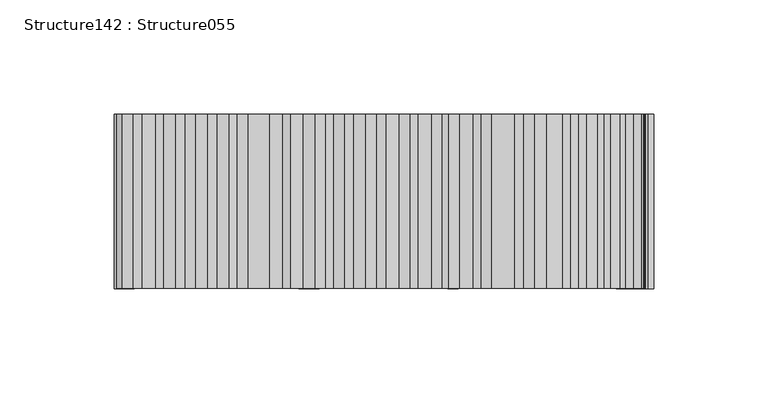
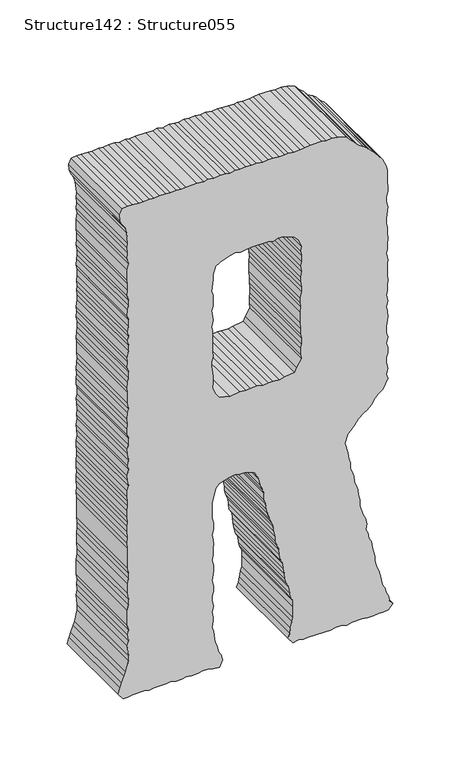
"""IFC4 building model written with IfcOpenShell, lengths in millimetres: proxy geometry, Structure142 : Structure055."""

from ifc_helpers import new_model, si_unit, frame, origin, place, context, project, spatial, polyline, outline, extrude, source, transform, mapped, element, save


def structure142_structure055_61f402d9(model_context):
    return source(origin(), model_context, "Body", "SweptSolid", [
        extrude(outline(polyline([(3899.7046941, -44803.696828), (3903.2059411, -44804.280904), (3907.888177, -44804.280904), (3918.4480792, -44803.1063335), (3923.1319197, -44804.280904), (3927.8077372, -44804.280904), (3932.4899731, -44803.1063335), (3936.0345445, -44803.1063335), (3941.8753048, -44803.696828), (3951.2606365, -44803.696828), (3955.360401, -44804.280904), (3962.9774586, -44807.7965925), (3967.6789497, -44811.3138855), (3970.5768654, -44813.6469805), (3974.1214368, -44817.7563726), (3977.6194746, -44820.679962), (3979.9621971, -44823.6244112), (3982.8793681, -44828.2986241), (3987.0048063, -44831.8143126), (3989.9460463, -44835.3396286), (3994.0233463, -44838.8601309), (3996.390138, -44845.8834848), (3997.5486624, -44851.1497967), (3996.9645864, -44855.8432649), (3997.5486624, -44859.9414248), (3997.5486624, -44869.9012049), (3996.9645864, -44874.594673), (3996.390138, -44878.1023385), (3996.390138, -44883.9703771), (3996.9645864, -44888.64459), (3996.390138, -44891.5890392), (3996.390138, -44896.2616475), (3996.9645864, -44902.1296862), (3996.9645864, -44905.6469792), (3996.390138, -44910.3404474), (3997.5486624, -44916.1908354), (3996.9645864, -44920.3002275), (3997.5486624, -44924.9824634), (3996.9645864, -44930.2487754), (3997.5486624, -44934.3485398), (3996.390138, -44939.042008), (3996.9645864, -44942.559301), (3997.5486624, -44947.2511646), (3996.390138, -44952.5190811), (3997.5486624, -44957.7934161), (3996.390138, -44961.3107092), (3996.9645864, -44967.1610972), (3996.9645864, -44976.5448243), (3996.390138, -44981.2286648), (3996.9645864, -44984.7443532), (3996.390138, -44990.0138744), (3996.9645864, -44994.1232665), (3996.9645864, -44999.3976015), (3996.390138, -45004.0798374), (3996.9645864, -45008.1715789), (3996.390138, -45013.4555415), (3996.390138, -45016.9664161), (3996.9645864, -45022.8312455), (3996.9645864, -45026.922987), (3996.390138, -45031.6164552), (3991.6806238, -45033.9655961), (3986.4046842, -45033.3847293), (3981.7208437, -45031.6164552), (3978.2035506, -45029.2753372), (3973.5197101, -45028.1007667), (3963.5615346, -45026.922987), (3959.4617701, -45027.5166907), (3954.7506513, -45026.922987), (3949.4923624, -45027.5166907), (3944.8165449, -45026.3485386), (3939.5325823, -45027.5166907), (3930.1745289, -45027.5166907), (3926.6492128, -45026.922987), (3920.7908018, -45026.922987), (3916.0909152, -45027.5166907), (3911.4054701, -45026.3485386), (3906.7328618, -45026.3485386), (3903.2059411, -45026.922987), (3897.3475301, -45027.5166907), (3893.822214, -45026.3485386), (3887.9621984, -45026.3485386), (3883.2863809, -45026.922987), (3878.5784713, -45026.3485386), (3875.0772243, -45026.922987), (3870.4030114, -45026.3485386), (3865.7015202, -45026.3485386), (3859.8591552, -45027.5166907), (3855.7353217, -45026.922987), (3850.4754282, -45027.5166907), (3846.3772683, -45026.3485386), (3841.0900965, -45026.3485386), (3836.9919366, -45026.922987), (3831.732043, -45027.5166907), (3828.2163546, -45026.922987), (3818.2309008, -45026.922987), (3812.9726119, -45026.3485386), (3809.4729695, -45026.922987), (3803.5872802, -45027.5166907), (3798.9050443, -45026.922987), (3794.8309535, -45027.5166907), (3789.5293402, -45027.5166907), (3786.0280932, -45026.3485386), (3780.1616592, -45026.3485386), (3776.6427615, -45027.5166907), (3771.9605256, -45026.922987), (3766.1021146, -45026.3485386), (3761.418274, -45026.922987), (3757.8753073, -45026.3485386), (3752.6170184, -45027.5166907), (3747.9428055, -45026.922987), (3742.6748889, -45026.3485386), (3738.5574738, -45027.5166907), (3733.2991849, -45027.5166907), (3729.1737467, -45026.922987), (3725.0996559, -45026.922987), (3720.4158154, -45027.5166907), (3714.5301261, -45027.5166907), (3709.8559132, -45026.922987), (3706.3289925, -45027.5166907), (3701.6547796, -45027.5166907), (3695.786741, -45026.922987), (3691.0868544, -45027.5166907), (3686.4030139, -45026.922987), (3668.2437048, -45026.922987), (3663.5598643, -45026.3485386), (3658.8840468, -45026.3485386), (3654.1841602, -45026.922987), (3645.4262289, -45026.922987), (3639.5405396, -45026.3485386), (3634.856699, -45026.3485386), (3630.1824862, -45027.5166907), (3616.69739, -45027.5166907), (3612.0135494, -45026.3485386), (3607.8961343, -45026.922987), (3602.0280957, -45026.3485386), (3597.9540049, -45027.5166907), (3588.5702778, -45026.3485386), (3583.8864372, -45026.3485386), (3574.5107332, -45028.6912612), (3570.9854171, -45029.8674363), (3565.7094775, -45032.1989266), (3561.6257591, -45033.3847293), (3556.3417965, -45035.1337482), (3551.0658569, -45031.0243561), (3551.0658569, -45026.922987), (3551.6675836, -45022.8312455), (3551.6675836, -45012.865047), (3551.0658569, -45008.7652825), (3551.6675836, -45004.0798374), (3551.6675836, -44994.1232665), (3552.242032, -44989.4297984), (3551.0658569, -44985.3380569), (3551.0658569, -44980.6461934), (3551.6675836, -44976.5448243), (3551.0658569, -44971.8513561), (3551.6675836, -44966.5866488), (3552.242032, -44962.4852797), (3552.242032, -44958.3758876), (3551.0658569, -44953.6936516), (3550.4833855, -44947.833636), (3556.3417965, -44945.4828904), (3561.6257591, -44946.6590655), (3565.1254015, -44949.0001835), (3570.9854171, -44950.1763586), (3574.5107332, -44951.9253775), (3585.0706354, -44953.099948), (3589.1527492, -44954.2777277), (3594.4286888, -44953.6936516), (3597.9540049, -44953.6936516), (3602.6298224, -44954.2777277), (3607.8961343, -44953.099948), (3613.1720739, -44954.2777277), (3617.2718384, -44954.2777277), (3621.3732075, -44953.099948), (3626.0554434, -44953.099948), (3631.915459, -44954.2777277), (3636.6153456, -44953.6936516), (3640.114988, -44953.099948), (3644.8245022, -44953.099948), (3650.1004418, -44954.2777277), (3654.1841602, -44953.6936516), (3660.0682449, -44953.6936516), (3664.7440624, -44953.099948), (3668.2437048, -44953.6936516), (3672.9435914, -44954.2777277), (3677.6274319, -44953.099948), (3683.4858429, -44953.099948), (3688.1873341, -44954.2777277), (3701.6547796, -44954.2777277), (3706.9130685, -44953.099948), (3713.9556777, -44951.3509291), (3717.4729707, -44948.4177121), (3719.8140887, -44940.2165785), (3720.9726131, -44934.3485398), (3719.8140887, -44930.8408744), (3719.8140887, -44924.9824634), (3716.8985223, -44917.9575049), (3709.2718371, -44913.8561358), (3703.4134261, -44912.6815653), (3698.711935, -44910.9148958), (3695.2122926, -44909.7467437), (3689.3458585, -44909.7467437), (3685.2444894, -44908.5721732), (3679.9701544, -44907.3959981), (3675.8687854, -44906.8151313), (3670.5848228, -44905.0645078), (3667.0851803, -44903.8787051), (3662.3836892, -44902.1296862), (3657.7014533, -44900.9551157), (3652.4431643, -44899.7789406), (3648.3161216, -44899.7789406), (3644.2420307, -44898.6123931), (3639.5405396, -44896.8553512), (3634.856699, -44896.2616475), (3629.5984101, -44895.6807807), (3625.472972, -44893.3380581), (3620.7971545, -44892.7539821), (3616.0972679, -44892.1634876), (3611.4134274, -44891.5890392), (3606.1551384, -44890.4112595), (3602.0280957, -44888.0621186), (3596.7698067, -44887.4876701), (3592.6700423, -44886.8955711), (3588.5702778, -44884.5464301), (3583.2863152, -44884.5464301), (3573.9266571, -44884.5464301), (3570.4109687, -44885.7210006), (3565.1254015, -44886.8955711), (3560.441561, -44887.4876701), (3556.3417965, -44889.236689), (3550.4833855, -44884.5464301), (3551.6675836, -44879.8706126), (3550.4833855, -44875.7612205), (3551.0658569, -44871.6598514), (3551.0658569, -44858.1763598), (3550.4833855, -44852.3275764), (3551.6675836, -44847.6341083), (3551.6675836, -44844.1248383), (3550.4833855, -44838.2664272), (3551.6675836, -44834.1666628), (3551.6675836, -44825.3734301), (3551.0658569, -44820.679962), (3551.0658569, -44815.41365), (3551.6675836, -44810.7233911), (3551.0658569, -44807.2044934), (3551.6675836, -44802.5222575), (3556.3417965, -44799.0049644), (3559.2669905, -44801.3541054), (3564.54293, -44802.5222575), (3568.0682461, -44804.280904), (3572.7440636, -44805.4538699), (3576.2693797, -44807.7965925), (3585.0706354, -44809.5456114), (3590.3289243, -44810.7233911), (3595.5872132, -44813.0629044), (3600.2967274, -44814.2390795), (3604.3964919, -44814.2390795), (3609.6547808, -44815.41365), (3613.772196, -44816.5882205), (3619.0385079, -44817.1642735), (3622.555801, -44819.5150191), (3627.8397636, -44820.1055136), (3631.3410106, -44821.8577417), (3636.6153456, -44821.264038), (3641.8832621, -44822.4386085), (3646.557475, -44824.7813311), (3654.7842823, -44827.1320766), (3660.6250426, -44827.1320766), (3665.3265338, -44828.2986241), (3670.0007467, -44828.8907232), (3674.1277895, -44830.055666), (3678.2018803, -44831.8143126), (3683.4858429, -44832.3983886), (3687.587212, -44833.5729591), (3691.6869765, -44835.3396286), (3696.9709391, -44835.3396286), (3701.0723082, -44836.5077807), (3706.9130685, -44837.6743282), (3716.2887726, -44840.0154461), (3723.9154578, -44837.6743282), (3726.2742264, -44834.7491342), (3729.7738688, -44831.8143126), (3734.47536, -44828.2986241), (3737.9750024, -44824.197255), (3739.7416719, -44821.264038), (3743.2332913, -44817.1642735), (3747.9428055, -44814.2390795), (3751.4424479, -44811.3138855), (3753.8012165, -44807.2044934), (3762.5848215, -44803.1063335), (3766.684586, -44804.280904), (3771.3860772, -44803.1063335), (3777.2444882, -44804.280904), (3781.9299333, -44804.280904), (3785.4456218, -44803.1063335), (3790.7039107, -44803.1063335), (3794.8309535, -44804.280904), (3800.0876378, -44803.1063335), (3804.1890069, -44804.280904), (3810.0474179, -44804.280904), (3818.2309008, -44803.1063335), (3823.5341187, -44803.696828), (3827.6162325, -44804.280904), (3832.8921721, -44803.1063335), (3838.1761347, -44804.280904), (3842.8583706, -44803.696828), (3846.9757858, -44803.696828), (3851.6612309, -44803.1063335), (3856.9179152, -44803.696828), (3866.8776953, -44803.696828), (3870.4030114, -44803.1063335), (3876.263027, -44804.280904), (3880.3627915, -44803.696828), (3884.4609514, -44803.696828), (3890.320967, -44803.1063335), (3894.4030808, -44803.696828), (3899.7046941, -44803.696828)]), holes=[polyline([(3794.8309535, -44930.8408744), (3793.6451507, -44939.042008), (3795.960595, -44947.833636), (3800.0876378, -44950.75883), (3805.9476534, -44953.6936516), (3811.7884138, -44953.099948), (3816.4883003, -44953.099948), (3820.5896694, -44953.6936516), (3825.849563, -44954.2777277), (3830.5574726, -44954.2777277), (3834.6588416, -44953.099948), (3839.9331766, -44953.6936516), (3858.1021133, -44953.6936516), (3861.6178018, -44954.2777277), (3867.4601667, -44953.099948), (3871.5599312, -44953.6936516), (3876.8438938, -44954.2777277), (3880.3627915, -44953.099948), (3890.320967, -44953.099948), (3894.4030808, -44954.2777277), (3904.9645876, -44953.099948), (3909.0627475, -44953.099948), (3916.0909152, -44950.75883), (3918.4480792, -44947.2511646), (3921.3748778, -44939.042008), (3922.5494483, -44934.3485398), (3921.3748778, -44929.6663039), (3921.9733953, -44926.1506155), (3922.5494483, -44920.3002275), (3922.5494483, -44905.6469792), (3921.3748778, -44900.9551157), (3922.5494483, -44897.4474503), (3922.5494483, -44892.7539821), (3919.0321552, -44883.9703771), (3915.5068392, -44880.4546886), (3908.46423, -44877.519867), (3904.3901392, -44878.1023385), (3900.2887701, -44877.519867), (3895.0048075, -44877.519867), (3890.905043, -44878.1023385), (3885.6210804, -44877.519867), (3880.9452629, -44878.1023385), (3876.8438938, -44878.1023385), (3871.5599312, -44877.519867), (3867.4601667, -44877.519867), (3862.2018778, -44878.6960421), (3858.1021133, -44878.6960421), (3854.0007442, -44878.1023385), (3849.3008577, -44878.6960421), (3839.9331766, -44878.6960421), (3834.0474873, -44878.1023385), (3829.374879, -44878.1023385), (3825.2911606, -44877.519867), (3820.015221, -44877.519867), (3816.4883003, -44878.1023385), (3810.6298893, -44878.1023385), (3806.5317294, -44877.519867), (3800.0876378, -44881.6196315), (3795.960595, -44883.378278), (3794.8309535, -44892.1634876), (3793.6451507, -44896.2616475), (3794.2292268, -44902.1296862), (3794.2292268, -44905.6469792), (3793.6451507, -44910.3404474), (3794.8309535, -44915.6067593), (3794.8309535, -44921.474798), (3794.2292268, -44924.9824634), (3794.8309535, -44930.8408744)])]), frame((0.0, 247945.1599557, 0.0), z_axis=(0.0, 1.0, 0.0), x_axis=(0.0, 0.0, 1.0)), (0.0, 0.0, 1.0), 76.2),
    ])


if __name__ == "__main__":
    model = new_model("IFC4")
    model_context = context("Model", 3, world=origin())
    ifc_project = project(units=[si_unit("LENGTHUNIT", "METRE", prefix="MILLI")], contexts=[model_context])
    site = spatial("IfcSite", under=ifc_project)
    building = spatial("IfcBuilding", under=site)
    placement = place(None, origin())
    structure142_structure055_shape = structure142_structure055_61f402d9(model_context)
    element("IfcBuildingElementProxy", 1, Name="Structure142 : Structure055", ObjectType="Structure142 : Structure055", at=placement, inside=building, context=model_context, shape_type="MappedRepresentation", body=[
        mapped(structure142_structure055_shape, transform((0.0, 0.0, 0.0), x_axis=(1.0, 0.0, 0.0), y_axis=(0.0, 1.0, 0.0), z_axis=(0.0, 0.0, 1.0))),
    ])
    save(model, "model.ifc")

# Revit data of these elements
# Type "Structure142 : Structure055"
#   NameOverride = "Structure055"
# Element 1 (IfcBuildingElementProxy, "Structure142 : Structure055")
#   Materials on its faces: "BRUSHED ALUM. LETTERING"
# Materials
#   "BRUSHED ALUM. LETTERING": class "Unassigned", colour RGB 169 181 186, transparency 0, Cost = 0
